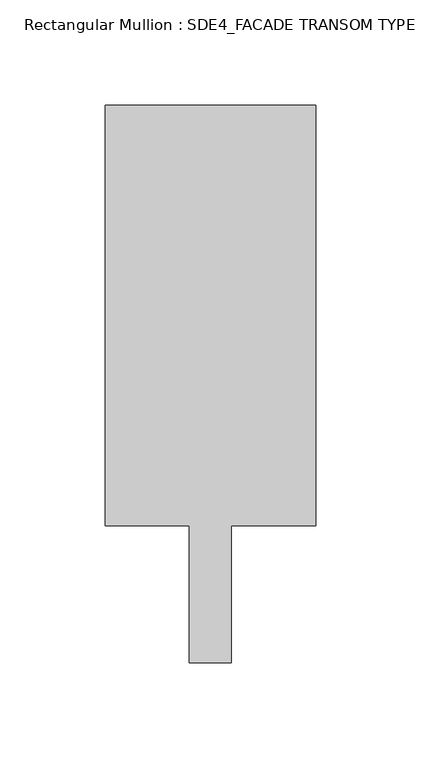
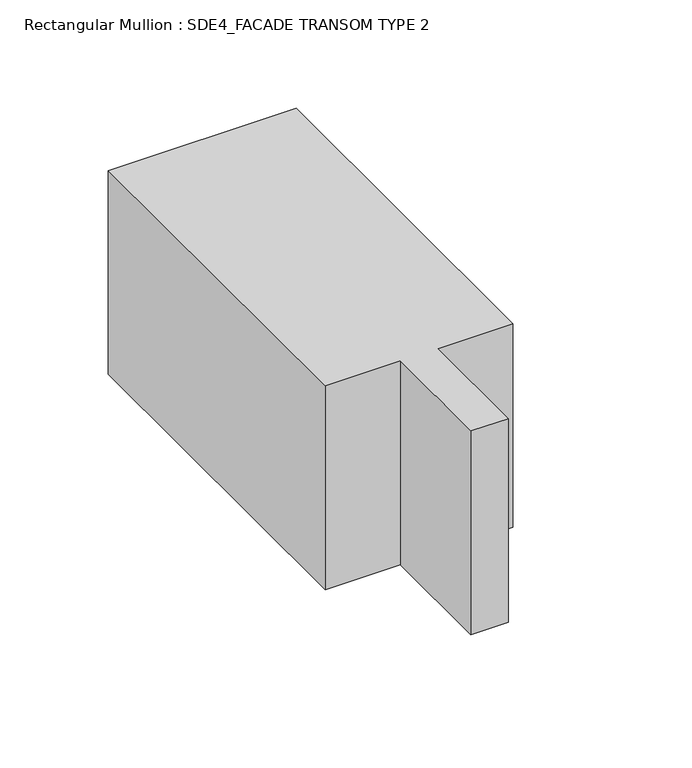
"""IFC4 building model written with IfcOpenShell, lengths in millimetres: member geometry, Rectangular Mullion : SDE4_FACADE TRANSOM TYPE 2."""

from ifc_helpers import new_model, si_unit, frame, origin, place, context, project, spatial, polyline, outline, extrude, source, transform, mapped, element, save


def rectangular_mullion_sde4_facade_transom_type_2_1c33c652(model_context):
    return source(origin(), model_context, "Body", "SweptSolid", [
        extrude(outline(polyline([(50.0, 132.5), (50.0, -67.5), (10.0, -67.5), (10.0, -132.5), (-10.0, -132.5), (-10.0, -67.5), (-50.0, -67.5), (-50.0, 132.5), (50.0, 132.5)])), frame((0.0, 0.0, -114.7995218), z_axis=(0.0, 0.0, 1.0), x_axis=(1.0, 0.0, 0.0)), (0.0, 0.0, 1.0), 114.7995218),
    ])


if __name__ == "__main__":
    model = new_model("IFC4")
    model_context = context("Model", 3, world=origin())
    ifc_project = project(units=[si_unit("LENGTHUNIT", "METRE", prefix="MILLI")], contexts=[model_context])
    site = spatial("IfcSite", under=ifc_project)
    building = spatial("IfcBuilding", under=site)
    placement = place(None, origin())
    rectangular_mullion_sde4_facade_transom_type_2_shape = rectangular_mullion_sde4_facade_transom_type_2_1c33c652(model_context)
    element("IfcMember", 1, ObjectType="Rectangular Mullion : SDE4_FACADE TRANSOM TYPE 2", at=placement, inside=building, context=model_context, shape_type="MappedRepresentation", body=[
        mapped(rectangular_mullion_sde4_facade_transom_type_2_shape, transform((0.0, 0.0, 0.0), x_axis=(1.0, 0.0, 0.0), y_axis=(0.0, 1.0, 0.0), z_axis=(0.0, 0.0, 1.0))),
    ])
    save(model, "model.ifc")

# Revit data of these elements
# Type "Rectangular Mullion : SDE4_FACADE TRANSOM TYPE 2"
#   built-in parameter 1007322 = 0.869423 (stored number, unit not read)
#   built-in parameter 1007321 = 0.164042 (stored number, unit not read)
#   built-in parameter 1007320 = 0.164042 (stored number, unit not read)
